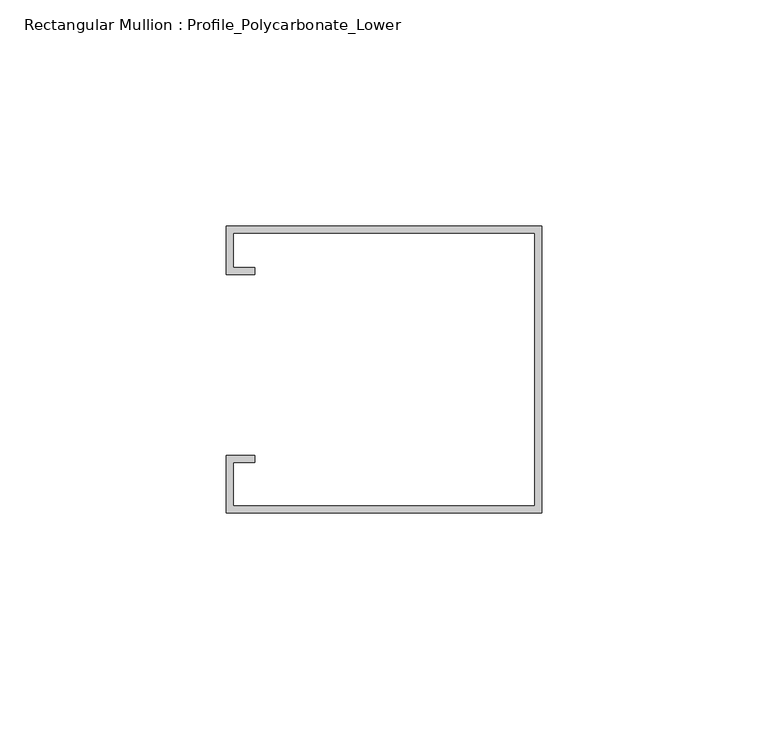
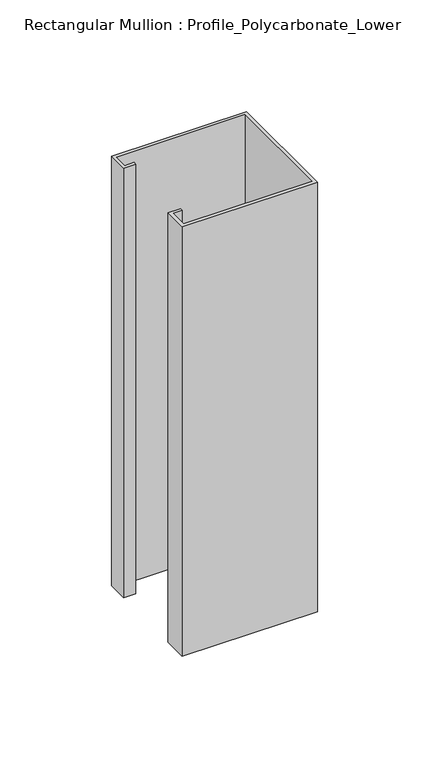
"""IFC4 building model written with IfcOpenShell, lengths in millimetres: member geometry, Rectangular Mullion : Profile_Polycarbonate_Lower."""

from ifc_helpers import new_model, si_unit, frame, origin, place, context, project, spatial, polyline, outline, extrude, source, transform, mapped, element, save


def rectangular_mullion_profile_polycarbonate_lower_1f1391b3(model_context):
    return source(origin(), model_context, "Body", "SweptSolid", [
        extrude(outline(polyline([(0.0, -32.7), (-69.85, -32.7), (-69.85, -20.0), (-63.5, -20.0), (-63.5, -21.5875), (-68.2625, -21.5875), (-68.2625, -31.1125), (-1.5875, -31.1125), (-1.5875, 29.2125), (-68.2625, 29.2125), (-68.2625, 21.5875), (-63.5, 21.5875), (-63.5, 20.0), (-69.85, 20.0), (-69.85, 30.8), (0.0, 30.8), (0.0, -32.7)])), frame((0.0, 0.0, -234.95), z_axis=(0.0, 0.0, 1.0), x_axis=(1.0, 0.0, 0.0)), (0.0, 0.0, 1.0), 234.95),
    ])


if __name__ == "__main__":
    model = new_model("IFC4")
    model_context = context("Model", 3, world=origin())
    ifc_project = project(units=[si_unit("LENGTHUNIT", "METRE", prefix="MILLI")], contexts=[model_context])
    site = spatial("IfcSite", under=ifc_project)
    building = spatial("IfcBuilding", under=site)
    placement = place(None, origin())
    rectangular_mullion_profile_polycarbonate_lower_shape = rectangular_mullion_profile_polycarbonate_lower_1f1391b3(model_context)
    element("IfcMember", 1, ObjectType="Rectangular Mullion : Profile_Polycarbonate_Lower", at=placement, inside=building, context=model_context, shape_type="MappedRepresentation", body=[
        mapped(rectangular_mullion_profile_polycarbonate_lower_shape, transform((0.0, 0.0, 0.0), x_axis=(1.0, 0.0, 0.0), y_axis=(0.0, 1.0, 0.0), z_axis=(0.0, 0.0, 1.0))),
    ])
    save(model, "model.ifc")

# Revit data of these elements
# Type "Rectangular Mullion : Profile_Polycarbonate_Lower"
#   built-in parameter 1007322 = 0.208333 (stored number, unit not read)
#   built-in parameter 1007321 = 0 (stored number, unit not read)
#   built-in parameter 1007320 = 0.00520833 (stored number, unit not read)
# Element 1 (IfcMember, "Rectangular Mullion : Profile_Polycarbonate_Lower")
#   Materials on its faces: "GALVANIZED UNISTRUT P5500, 1 5/8\" X 2 7/16\" OR ALUM. CHANNEL"
# Materials
#   "GALVANIZED UNISTRUT P5500, 1 5/8\" X 2 7/16\" OR ALUM. CHANNEL": class "Metal", colour RGB 244 244 244, transparency 0, Description = "Aluminum 6061", Cost = 0
